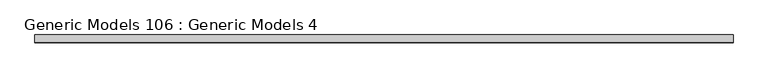
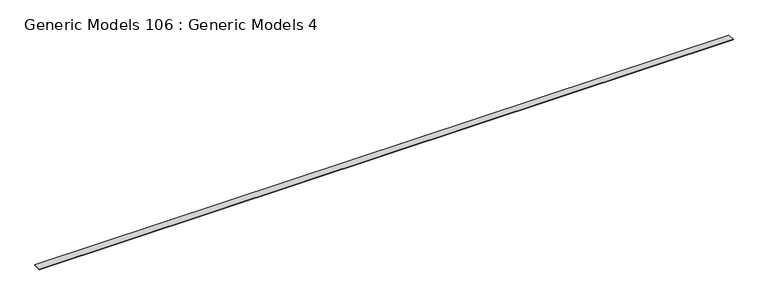
"""IFC4 building model written with IfcOpenShell, lengths in millimetres: proxy geometry, Generic Models 106 : Generic Models 4."""

from ifc_helpers import new_model, si_unit, frame, origin, place, context, project, spatial, polyline, outline, extrude, source, transform, mapped, element, save


def generic_models_106_generic_models_4_1e1792a3(model_context):
    return source(origin(), model_context, "Body", "SweptSolid", [
        extrude(outline(polyline([(0.0, -211.2582119), (0.0, 0.0), (18643.6, 0.0), (18643.6, -211.2582119), (0.0, -211.2582119)])), frame((-2152.1733045, 51483.8113896, 126956.9275355), z_axis=(0.0, 0.020828813681927037, 0.9997830567281102), x_axis=(-1.0, 0.0, 0.0)), (0.0, 0.0, 1.0), 12.7),
    ])


if __name__ == "__main__":
    model = new_model("IFC4")
    model_context = context("Model", 3, world=origin())
    ifc_project = project(units=[si_unit("LENGTHUNIT", "METRE", prefix="MILLI")], contexts=[model_context])
    site = spatial("IfcSite", under=ifc_project)
    building = spatial("IfcBuilding", under=site)
    placement = place(None, origin())
    generic_models_106_generic_models_4_shape = generic_models_106_generic_models_4_1e1792a3(model_context)
    element("IfcBuildingElementProxy", 1, Name="Generic Models 106 : Generic Models 4", ObjectType="Generic Models 106 : Generic Models 4", at=placement, inside=building, context=model_context, shape_type="MappedRepresentation", body=[
        mapped(generic_models_106_generic_models_4_shape, transform((0.0, 0.0, 0.0), x_axis=(1.0, 0.0, 0.0), y_axis=(0.0, 1.0, 0.0), z_axis=(0.0, 0.0, 1.0))),
    ])
    save(model, "model.ifc")

# Revit data of these elements
# Element 1 (IfcBuildingElementProxy, "Generic Models 106 : Generic Models 4")
#   Materials on its faces: "_1/2\" CDX PLYWOOD"
# Materials
#   "_1/2\" CDX PLYWOOD": class "Generic", colour RGB 98 75 74, transparency 0, Cost = 0
